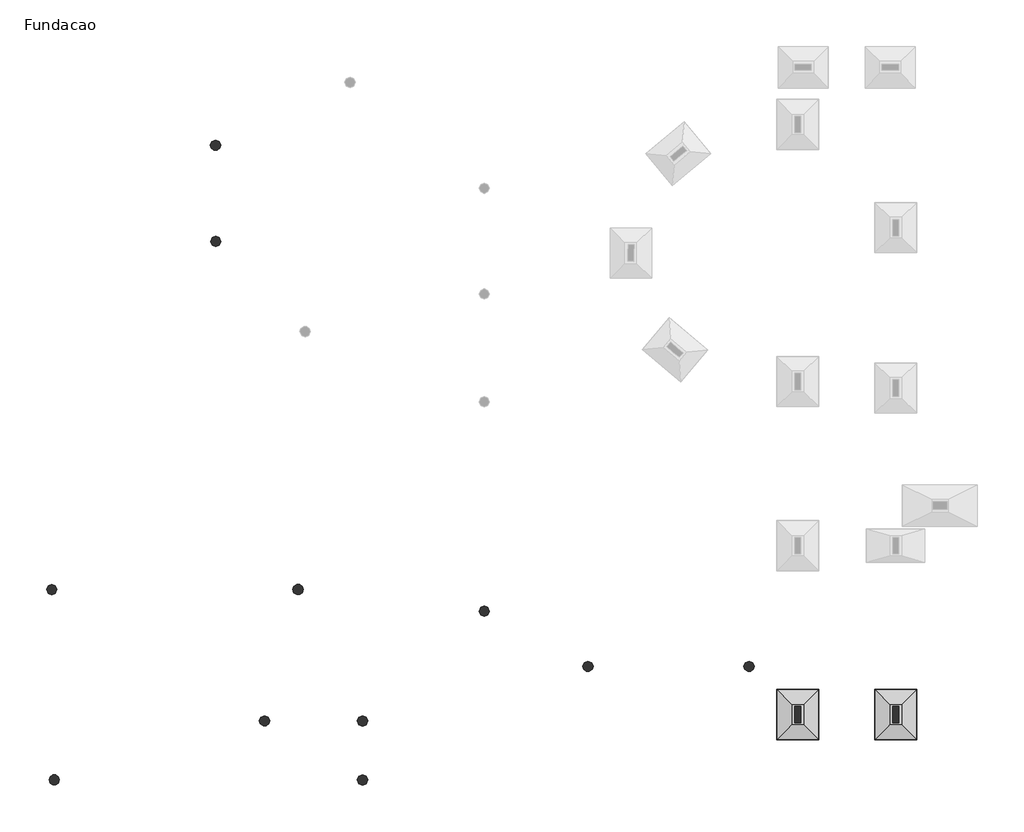
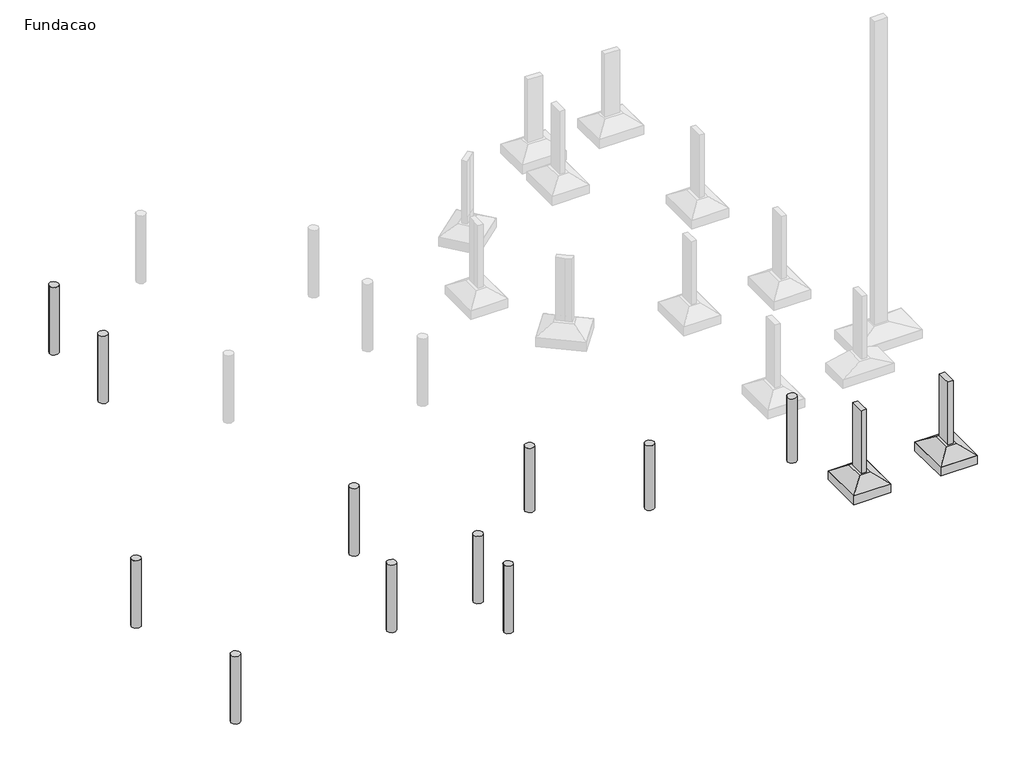
# One storey, part 1 of 2: 13 columns, 2 fasteners.
"""IFC4 building model written with IfcOpenShell, lengths in millimetres."""

import ifcopenshell
import ifcopenshell.guid

model = None  # the IFC model being written
_history = None  # IfcOwnerHistory: only IFC2X3 demands one
_inside = {}  # id of a spatial element -> (the spatial element, [elements in it])
_under = {}  # id of a project, library or spatial element -> (it, [spatial elements below it])
_declared = {}  # id of a project -> (the project, [libraries it declares])
_typed = {}  # id of a type object -> (the type object, [elements of that type])
_made_of = {}  # id of a material, layer set ... -> (it, [elements and type objects made of it])


def new_model(schema):
    """Start an empty IFC model of exactly this schema.

    Asked for "IFC4X3", IfcOpenShell would pick the latest addendum, in which some entities
    have other attributes; the version numbers below select the first issue.
    IFC2X3 requires an IfcOwnerHistory on every rooted entity: one is made here for all.
    """
    global model, _history
    if schema == "IFC4X3":
        model = ifcopenshell.file(schema_version=(4, 3, 0, 0))
    else:
        model = ifcopenshell.file(schema=schema)
    _inside.clear()
    _under.clear()
    _declared.clear()
    _typed.clear()
    _made_of.clear()
    _history = None
    if model.schema == "IFC2X3":
        org = make("IfcOrganization", Name="unknown")
        user = make(
            "IfcPersonAndOrganization",
            ThePerson=make("IfcPerson", FamilyName="unknown"),
            TheOrganization=org,
        )
        app = make(
            "IfcApplication",
            ApplicationDeveloper=org,
            Version="unknown",
            ApplicationFullName="unknown",
            ApplicationIdentifier="unknown",
        )
        _history = make(
            "IfcOwnerHistory",
            OwningUser=user,
            OwningApplication=app,
            ChangeAction="ADDED",
            CreationDate=0,
        )
    return model


def make(cls, **values):
    """One entity of the class cls with the attributes given. An attribute that is None is left unset."""
    return model.create_entity(
        cls, **{name: value for name, value in values.items() if value is not None}
    )


def rooted(cls, **values):
    """An entity with a GlobalId (a new one), such as an element, a storey or a relation."""
    return make(cls, GlobalId=ifcopenshell.guid.new(), OwnerHistory=_history, **values)


def si_unit(unit_type, name, prefix=None):
    """IfcSIUnit, for example si_unit("LENGTHUNIT", "METRE", prefix="MILLI")."""
    return make("IfcSIUnit", UnitType=unit_type, Prefix=prefix, Name=name)


def assignment(units):
    """IfcUnitAssignment: the units of a project."""
    return None if units is None else make("IfcUnitAssignment", Units=units)


def point(xyz):
    """IfcCartesianPoint."""
    return None if xyz is None else make("IfcCartesianPoint", Coordinates=xyz)


def direction(xyz):
    """IfcDirection."""
    return None if xyz is None else make("IfcDirection", DirectionRatios=xyz)


def frame(location, z_axis=None, x_axis=None):
    """IfcAxis2Placement3D, a coordinate frame: its origin and axes. An axis left out is left unset."""
    return make(
        "IfcAxis2Placement3D",
        Location=point(location),
        Axis=direction(z_axis),
        RefDirection=direction(x_axis),
    )


def origin():
    """The frame at (0, 0, 0) with its axes left unset."""
    return frame((0.0, 0.0, 0.0))


def place(relative_to, where):
    """IfcLocalPlacement: puts the frame where relative to a parent placement (None: the world)."""
    return make(
        "IfcLocalPlacement", PlacementRelTo=relative_to, RelativePlacement=where
    )


def context(
    kind, dimensions, precision=None, world=None, true_north=None, identifier=None
):
    """IfcGeometricRepresentationContext, for example the 3D "Model" context."""
    return make(
        "IfcGeometricRepresentationContext",
        ContextIdentifier=identifier,
        ContextType=kind,
        CoordinateSpaceDimension=dimensions,
        Precision=precision,
        WorldCoordinateSystem=world,
        TrueNorth=true_north,
    )


def project(units=None, contexts=None):
    """IfcProject with its units and contexts."""
    return rooted(
        "IfcProject",
        Name="project",
        RepresentationContexts=contexts,
        UnitsInContext=assignment(units),
    )


def spatial(cls, under=None, at=None, **own):
    """A site, building, storey or space (cls), placed at a placement, below another one or the project."""
    s = rooted(cls, ObjectPlacement=at, **own)
    if under is not None:
        _under.setdefault(under.id(), (under, []))[1].append(s)
    return s


def polyline(points):
    """IfcPolyline through the points."""
    return make("IfcPolyline", Points=[point(p) for p in points])


def circle_curve(where, radius):
    """IfcCircle in the frame where."""
    return make("IfcCircle", Position=where, Radius=radius)


def outline(outer, holes=None, kind="AREA"):
    """IfcArbitraryClosedProfileDef: a profile drawn as a closed curve; with holes, ...WithVoids."""
    if holes is None:
        return make("IfcArbitraryClosedProfileDef", ProfileType=kind, OuterCurve=outer)
    return make(
        "IfcArbitraryProfileDefWithVoids",
        ProfileType=kind,
        OuterCurve=outer,
        InnerCurves=holes,
    )


def extrude(swept, where, along, depth):
    """IfcExtrudedAreaSolid: the profile swept, set in the frame where, extruded along a direction by depth."""
    return make(
        "IfcExtrudedAreaSolid",
        SweptArea=swept,
        Position=where,
        ExtrudedDirection=direction(along),
        Depth=depth,
    )


def faces_of(points, faces, orient=None, outer=None):
    """IfcFace entities. A face is a list of loops; a loop is a list of indices into points, from 0.

    orient and outer hold one flag for each loop. By default every Orientation is true, the
    first loop of a face is its IfcFaceOuterBound and the others are IfcFaceBound.
    """
    made = []
    for i, loops in enumerate(faces):
        bounds = []
        for j, loop in enumerate(loops):
            is_outer = j == 0 if outer is None else outer[i][j]
            bounds.append(
                make(
                    "IfcFaceOuterBound" if is_outer else "IfcFaceBound",
                    Bound=make("IfcPolyLoop", Polygon=[points[k] for k in loop]),
                    Orientation=True if orient is None else orient[i][j],
                )
            )
        made.append(make("IfcFace", Bounds=bounds))
    return made


def faceted_brep(points, faces, orient=None, outer=None, voids=None):
    """IfcFacetedBrep: a solid bounded by flat faces; with voids (closed shells), ...WithVoids."""
    shared = [point(p) for p in points]
    hull = make("IfcClosedShell", CfsFaces=faces_of(shared, faces, orient, outer))
    if voids is None:
        return make("IfcFacetedBrep", Outer=hull)
    return make(
        "IfcFacetedBrepWithVoids",
        Outer=hull,
        Voids=[
            make(cls, CfsFaces=faces_of(shared, fs, o, b)) for cls, fs, o, b in voids
        ],
    )


def shape(context_of_items, identifier, shape_type, items):
    """IfcShapeRepresentation: the items that make up one representation, for example the "Body"."""
    return make(
        "IfcShapeRepresentation",
        ContextOfItems=context_of_items,
        RepresentationIdentifier=identifier,
        RepresentationType=shape_type,
        Items=items,
    )


def source(mapping_origin, context_of_items, identifier, shape_type, items):
    """IfcRepresentationMap: a shape defined once, which mapped items show again and again."""
    return make(
        "IfcRepresentationMap",
        MappingOrigin=mapping_origin,
        MappedRepresentation=shape(context_of_items, identifier, shape_type, items),
    )


def transform(
    local_origin,
    x_axis=None,
    y_axis=None,
    z_axis=None,
    scale=None,
    scale2=None,
    scale3=None,
    uniform=True,
):
    """IfcCartesianTransformationOperator3D, or its non-uniform kind. x_axis, y_axis, z_axis: its Axis1, 2, 3."""
    if uniform:
        return make(
            "IfcCartesianTransformationOperator3D",
            Axis1=direction(x_axis),
            Axis2=direction(y_axis),
            LocalOrigin=point(local_origin),
            Scale=scale,
            Axis3=direction(z_axis),
        )
    return make(
        "IfcCartesianTransformationOperator3DnonUniform",
        Axis1=direction(x_axis),
        Axis2=direction(y_axis),
        LocalOrigin=point(local_origin),
        Scale=scale,
        Axis3=direction(z_axis),
        Scale2=scale2,
        Scale3=scale3,
    )


def mapped(mapping_source, mapping_target):
    """IfcMappedItem: shows the shape of a source again, moved by a transform."""
    return make(
        "IfcMappedItem", MappingSource=mapping_source, MappingTarget=mapping_target
    )


def made_of(thing, what):
    """Note that an element or type object is made of a material, layer set ...; save() writes the relation."""
    if what is not None:
        _made_of.setdefault(what.id(), (what, []))[1].append(thing)
    return thing


def element(
    cls,
    number,
    at=None,
    inside=None,
    cuts=None,
    type_object=None,
    material=None,
    context=None,
    identifier="Body",
    shape_type=None,
    held_by="IfcProductDefinitionShape",
    body=None,
    shapes=None,
    **own,
):
    """One element of the class cls, such as IfcWall. Its Tag is "e" and its number.

    at: its placement. inside: the storey or other place that contains it. cuts: it is an
    opening in that element (IfcRelVoidsElement). A single representation is given by context,
    identifier, shape_type and body (its items); several are given by shapes. held_by: the class
    of the entity that holds the representations. save() writes the other relations.
    """
    e = rooted(cls, Tag="e%d" % number, ObjectPlacement=at, **own)
    if body is not None:
        shapes = [shape(context, identifier, shape_type, body)]
    if shapes is not None:
        e.Representation = make(held_by, Representations=shapes)
    if inside is not None:
        _inside.setdefault(inside.id(), (inside, []))[1].append(e)
    if cuts is not None:
        rooted(
            "IfcRelVoidsElement", RelatingBuildingElement=cuts, RelatedOpeningElement=e
        )
    if type_object is not None:
        _typed.setdefault(type_object.id(), (type_object, []))[1].append(e)
    return made_of(e, material)


def aggregate(whole, parts):
    """IfcRelAggregates: a whole, such as a stair, and the parts it consists of."""
    return rooted("IfcRelAggregates", RelatingObject=whole, RelatedObjects=parts)


def save(model, path):
    """Write the relations noted so far, then the file.

    IfcRelAggregates (storeys below a building ...), IfcRelContainedInSpatialStructure (elements
    in a storey), IfcRelDefinesByType, IfcRelAssociatesMaterial and IfcRelDeclares: one each for
    every whole, place, type object, material and project.
    """
    for whole, parts in _under.values():
        aggregate(whole, parts)
    for where, things in _inside.values():
        rooted(
            "IfcRelContainedInSpatialStructure",
            RelatedElements=things,
            RelatingStructure=where,
        )
    for kind, things in _typed.values():
        rooted("IfcRelDefinesByType", RelatedObjects=things, RelatingType=kind)
    for what, things in _made_of.values():
        rooted("IfcRelAssociatesMaterial", RelatedObjects=things, RelatingMaterial=what)
    for by, libraries in _declared.values():
        rooted("IfcRelDeclares", RelatingContext=by, RelatedDefinitions=libraries)
    model.write(path)


def plane_surface(at):
    """IfcPlane: the flat surface through the origin of the frame at, square to its z axis."""
    return make("IfcPlane", Position=at)


def cylinder_surface(at, radius):
    """IfcCylindricalSurface: all points at the distance radius from the z axis of the frame at."""
    return make("IfcCylindricalSurface", Position=at, Radius=radius)


def advanced_brep(points, edges, surfaces, faces):
    """IfcAdvancedBrep: a solid bounded by faces that lie on surfaces and meet in shared edges.

    An edge is (start, end): straight between two places in points (the first is 0);
    or (start, end, curve); or (start, end, curve, False) where it runs against its curve.
    A face is (place in surfaces, loops), or (place, loops, False) where it looks against
    its surface's normal. A loop lists edges by number (the first is 1), with a minus sign
    where the edge is run from its end to its start. The first loop is the outer one.
    """
    corners = [point(p) for p in points]
    vertices = [make("IfcVertexPoint", VertexGeometry=c) for c in corners]
    made = []
    for start, end, *more in edges:
        made.append(
            make(
                "IfcEdgeCurve",
                EdgeStart=vertices[start],
                EdgeEnd=vertices[end],
                EdgeGeometry=more[0] if more else make("IfcPolyline", Points=[corners[start], corners[end]]),
                SameSense=more[1] if len(more) > 1 else True,
            )
        )
    hull = []
    for where, loops, *sense in faces:
        bounds = []
        for j, loop in enumerate(loops):
            ring = [make("IfcOrientedEdge", EdgeElement=made[abs(k) - 1], Orientation=k > 0) for k in loop]
            bounds.append(
                make(
                    "IfcFaceOuterBound" if j == 0 else "IfcFaceBound",
                    Bound=make("IfcEdgeLoop", EdgeList=ring),
                    Orientation=True,
                )
            )
        hull.append(make("IfcAdvancedFace", Bounds=bounds, FaceSurface=surfaces[where], SameSense=sense[0] if sense else True))
    return make("IfcAdvancedBrep", Outer=make("IfcClosedShell", CfsFaces=hull))


def sps1_6b3be553(model_context):
    return source(origin(), model_context, "Body", "SolidModel", [
        faceted_brep([(-55.0, 50.0, 0.0), (-345.0, 50.0, 0.0), (-345.0, -450.0, 0.0), (-55.0, -450.0, 0.0), (300.0, 400.0, -250.0), (300.0, -800.0, -250.0), (-700.0, -800.0, -250.0), (-700.0, 400.0, -250.0)], [[[0, 1, 2, 3]], [[4, 5, 6, 7]], [[4, 7, 1, 0]], [[7, 6, 2, 1]], [[6, 5, 3, 2]], [[5, 4, 0, 3]]]),
        extrude(outline(polyline([(300.0, 400.0), (300.0, -800.0), (-700.0, -800.0), (-700.0, 400.0), (300.0, 400.0)])), frame((0.0, 0.0, -500.0), z_axis=(0.0, 0.0, 1.0), x_axis=(1.0, 0.0, 0.0)), (0.0, 0.0, 1.0), 250.0),
    ])


model = new_model("IFC4")

# Units and contexts
model_context = context("Model", 3, world=origin())
ifc_project = project(units=[si_unit("LENGTHUNIT", "METRE", prefix="MILLI")], contexts=[model_context])

# Site, building, storey
site = spatial("IfcSite", under=ifc_project)
building = spatial("IfcBuilding", under=site)
storey = spatial("IfcBuildingStorey", under=building, Name="Fundacao", Elevation=-1200.0)

# Columns
placement = place(None, origin())
element("IfcColumn", 1, ObjectType="TQS - Pilar circular : TQS - Pilar circular 25.0cm", at=placement, inside=storey, context=model_context, shape_type="AdvancedBrep", body=[
    advanced_brep(
    [(1325.0, -5454.2, -1500.0), (1575.0, -5454.2, -1500.0), (1325.0, -5454.2, 430.0), (1368.7596159, -5359.2, 430.0), (1575.0, -5454.2, 430.0), (1368.759616, -5549.2, 430.0)],
    [
        (0, 1, circle_curve(frame((1450.0, -5454.2, -1500.0), z_axis=(0.0, 0.0, -1.0), x_axis=(1.0, 0.0, 0.0)), 125.0)),
        (1, 0, circle_curve(frame((1450.0, -5454.2, -1500.0), z_axis=(0.0, 0.0, -1.0), x_axis=(1.0, 0.0, 0.0)), 125.0)),
        (2, 3, circle_curve(frame((1450.0, -5454.2, 430.0), z_axis=(0.0, 0.0, -1.0), x_axis=(1.0, 0.0, 0.0)), 125.0)),
        (3, 4, circle_curve(frame((1450.0, -5454.2, 430.0), z_axis=(0.0, 0.0, -1.0), x_axis=(1.0, 0.0, 0.0)), 125.0)),
        (4, 1),
        (0, 2),
        (4, 5, circle_curve(frame((1450.0, -5454.2, 430.0), z_axis=(0.0, 0.0, -1.0), x_axis=(1.0, 0.0, 0.0)), 125.0)),
        (5, 2, circle_curve(frame((1450.0, -5454.2, 430.0), z_axis=(0.0, 0.0, -1.0), x_axis=(1.0, 0.0, 0.0)), 125.0)),
    ],
    [
        plane_surface(frame((1575.0, -5454.2, -1500.0), z_axis=(0.0, 0.0, -1.0), x_axis=(0.0, -1.0, 0.0))),
        cylinder_surface(frame((1450.0, -5454.2, -1500.0), z_axis=(0.0, 0.0, 1.0), x_axis=(1.0, 0.0, 0.0)), 125.0),
        plane_surface(frame((1575.0, -5454.2, 430.0), z_axis=(0.0, 0.0, 1.0), x_axis=(0.0, 1.0, 0.0))),
    ],
    [
        (0, [[1, 2]]),
        (1, [[3, 4, 5, -1, 6]]),
        (1, [[7, 8, -6, -2, -5]]),
        (2, [[-8, -7, -4, -3]]),
    ],
),
])
element("IfcColumn", 2, ObjectType="TQS - Pilar circular : TQS - Pilar circular 25.0cm", at=placement, inside=storey, context=model_context, shape_type="AdvancedBrep", body=[
    advanced_brep(
    [(1325.0, -4039.0, -1500.0), (1575.0, -4039.0, -1500.0), (1325.0, -4039.0, 430.0), (1346.4384241, -3969.0, 430.0), (1575.0, -4039.0, 430.0), (1346.4384241, -4109.0, 430.0)],
    [
        (0, 1, circle_curve(frame((1450.0, -4039.0, -1500.0), z_axis=(0.0, 0.0, -1.0), x_axis=(1.0, 0.0, 0.0)), 125.0)),
        (1, 0, circle_curve(frame((1450.0, -4039.0, -1500.0), z_axis=(0.0, 0.0, -1.0), x_axis=(1.0, 0.0, 0.0)), 125.0)),
        (2, 3, circle_curve(frame((1450.0, -4039.0, 430.0), z_axis=(0.0, 0.0, -1.0), x_axis=(1.0, 0.0, 0.0)), 125.0)),
        (3, 4, circle_curve(frame((1450.0, -4039.0, 430.0), z_axis=(0.0, 0.0, -1.0), x_axis=(1.0, 0.0, 0.0)), 125.0)),
        (4, 1),
        (0, 2),
        (4, 5, circle_curve(frame((1450.0, -4039.0, 430.0), z_axis=(0.0, 0.0, -1.0), x_axis=(1.0, 0.0, 0.0)), 125.0)),
        (5, 2, circle_curve(frame((1450.0, -4039.0, 430.0), z_axis=(0.0, 0.0, -1.0), x_axis=(1.0, 0.0, 0.0)), 125.0)),
    ],
    [
        plane_surface(frame((1575.0, -4039.0, -1500.0), z_axis=(0.0, 0.0, -1.0), x_axis=(0.0, -1.0, 0.0))),
        cylinder_surface(frame((1450.0, -4039.0, -1500.0), z_axis=(0.0, 0.0, 1.0), x_axis=(1.0, 0.0, 0.0)), 125.0),
        plane_surface(frame((1575.0, -4039.0, 430.0), z_axis=(0.0, 0.0, 1.0), x_axis=(0.0, 1.0, 0.0))),
    ],
    [
        (0, [[1, 2]]),
        (1, [[3, 4, 5, -1, 6]]),
        (1, [[7, 8, -6, -2, -5]]),
        (2, [[-8, -7, -4, -3]]),
    ],
),
])
element("IfcColumn", 3, ObjectType="TQS - Pilar circular : TQS - Pilar circular 25.0cm", at=placement, inside=storey, context=model_context, shape_type="AdvancedBrep", body=[
    advanced_brep(
    [(-6065.0, -5454.2, -1500.0), (-5815.0, -5454.2, -1500.0), (-6065.0, -5454.2, 430.0), (-6021.218638, -5359.181408, 430.0), (-5930.0226515, -5329.5988262, 430.0), (-5858.759616, -5359.2, 430.0), (-5815.0, -5454.2, 430.0), (-5858.759616, -5549.2, 430.0), (-6021.218638, -5549.218592, 430.0)],
    [
        (0, 1, circle_curve(frame((-5940.0, -5454.2, -1500.0), z_axis=(0.0, 0.0, -1.0), x_axis=(1.0, 0.0, 0.0)), 125.0)),
        (1, 0, circle_curve(frame((-5940.0, -5454.2, -1500.0), z_axis=(0.0, 0.0, -1.0), x_axis=(1.0, 0.0, 0.0)), 125.0)),
        (2, 3, circle_curve(frame((-5940.0, -5454.2, 430.0), z_axis=(0.0, 0.0, -1.0), x_axis=(1.0, 0.0, 0.0)), 125.0)),
        (3, 4, circle_curve(frame((-5940.0, -5454.2, 430.0), z_axis=(0.0, 0.0, -1.0), x_axis=(1.0, 0.0, 0.0)), 125.0)),
        (4, 5, circle_curve(frame((-5940.0, -5454.2, 430.0), z_axis=(0.0, 0.0, -1.0), x_axis=(1.0, 0.0, 0.0)), 125.0)),
        (5, 6, circle_curve(frame((-5940.0, -5454.2, 430.0), z_axis=(0.0, 0.0, -1.0), x_axis=(1.0, 0.0, 0.0)), 125.0)),
        (6, 1),
        (0, 2),
        (6, 7, circle_curve(frame((-5940.0, -5454.2, 430.0), z_axis=(0.0, 0.0, -1.0), x_axis=(1.0, 0.0, 0.0)), 125.0)),
        (7, 8, circle_curve(frame((-5940.0, -5454.2, 430.0), z_axis=(0.0, 0.0, -1.0), x_axis=(1.0, 0.0, 0.0)), 125.0)),
        (8, 2, circle_curve(frame((-5940.0, -5454.2, 430.0), z_axis=(0.0, 0.0, -1.0), x_axis=(1.0, 0.0, 0.0)), 125.0)),
    ],
    [
        plane_surface(frame((-5815.0, -5454.2, -1500.0), z_axis=(0.0, 0.0, -1.0), x_axis=(0.0, -1.0, 0.0))),
        cylinder_surface(frame((-5940.0, -5454.2, -1500.0), z_axis=(0.0, 0.0, 1.0), x_axis=(1.0, 0.0, 0.0)), 125.0),
        plane_surface(frame((-5815.0, -5454.2, 430.0), z_axis=(0.0, 0.0, 1.0), x_axis=(0.0, 1.0, 0.0))),
    ],
    [
        (0, [[1, 2]]),
        (1, [[3, 4, 5, 6, 7, -1, 8]]),
        (1, [[9, 10, 11, -8, -2, -7]]),
        (2, [[-11, -10, -9, -6, -5, -4, -3]]),
    ],
),
])
element("IfcColumn", 4, ObjectType="TQS - Pilar circular : TQS - Pilar circular 25.0cm", at=placement, inside=storey, context=model_context, shape_type="AdvancedBrep", body=[
    advanced_brep(
    [(4239.0, -1407.1, -1500.0), (4489.0, -1407.1, -1500.0), (4239.0, -1407.1, 340.0), (4269.0, -1325.859616, 340.0), (4459.0, -1325.859616, 340.0), (4489.0, -1407.1, 340.0), (4459.0, -1488.340384, 340.0), (4269.0, -1488.340384, 340.0)],
    [
        (0, 1, circle_curve(frame((4364.0, -1407.1, -1500.0), z_axis=(0.0, 0.0, -1.0), x_axis=(1.0, 0.0, 0.0)), 125.0)),
        (1, 0, circle_curve(frame((4364.0, -1407.1, -1500.0), z_axis=(0.0, 0.0, -1.0), x_axis=(1.0, 0.0, 0.0)), 125.0)),
        (2, 3, circle_curve(frame((4364.0, -1407.1, 340.0), z_axis=(0.0, 0.0, -1.0), x_axis=(1.0, 0.0, 0.0)), 125.0)),
        (3, 4, circle_curve(frame((4364.0, -1407.1, 340.0), z_axis=(0.0, 0.0, -1.0), x_axis=(1.0, 0.0, 0.0)), 125.0)),
        (4, 5, circle_curve(frame((4364.0, -1407.1, 340.0), z_axis=(0.0, 0.0, -1.0), x_axis=(1.0, 0.0, 0.0)), 125.0)),
        (5, 1),
        (0, 2),
        (5, 6, circle_curve(frame((4364.0, -1407.1, 340.0), z_axis=(0.0, 0.0, -1.0), x_axis=(1.0, 0.0, 0.0)), 125.0)),
        (6, 7, circle_curve(frame((4364.0, -1407.1, 340.0), z_axis=(0.0, 0.0, -1.0), x_axis=(1.0, 0.0, 0.0)), 125.0)),
        (7, 2, circle_curve(frame((4364.0, -1407.1, 340.0), z_axis=(0.0, 0.0, -1.0), x_axis=(1.0, 0.0, 0.0)), 125.0)),
    ],
    [
        plane_surface(frame((4489.0, -1407.1, -1500.0), z_axis=(0.0, 0.0, -1.0), x_axis=(0.0, -1.0, 0.0))),
        cylinder_surface(frame((4364.0, -1407.1, -1500.0), z_axis=(0.0, 0.0, 1.0), x_axis=(1.0, 0.0, 0.0)), 125.0),
        plane_surface(frame((4489.0, -1407.1, 340.0), z_axis=(0.0, 0.0, 1.0), x_axis=(0.0, 1.0, 0.0))),
    ],
    [
        (0, [[1, 2]]),
        (1, [[3, 4, 5, 6, -1, 7]]),
        (1, [[8, 9, 10, -7, -2, -6]]),
        (2, [[-10, -9, -8, -5, -4, -3]]),
    ],
),
])
element("IfcColumn", 5, ObjectType="TQS - Pilar circular : TQS - Pilar circular 25.0cm", at=placement, inside=storey, context=model_context, shape_type="AdvancedBrep", body=[
    advanced_brep(
    [(-6125.0, -889.0, -1500.0), (-5875.0, -889.0, -1500.0), (-6125.0, -889.0, 430.0), (-6103.5615759, -819.0, 430.0), (-6069.9643265, -785.4143204, 430.0), (-5929.9854905, -785.448233, 430.0), (-5896.4557386, -818.9743909, 430.0), (-5875.0, -889.0, 430.0), (-5896.4557386, -959.0256091, 430.0), (-5929.9854905, -992.551767, 430.0), (-6069.9643265, -992.5856796, 430.0), (-6103.5615759, -959.0, 430.0)],
    [
        (0, 1, circle_curve(frame((-6000.0, -889.0, -1500.0), z_axis=(0.0, 0.0, -1.0), x_axis=(1.0, 0.0, 0.0)), 125.0)),
        (1, 0, circle_curve(frame((-6000.0, -889.0, -1500.0), z_axis=(0.0, 0.0, -1.0), x_axis=(1.0, 0.0, 0.0)), 125.0)),
        (2, 3, circle_curve(frame((-6000.0, -889.0, 430.0), z_axis=(0.0, 0.0, -1.0), x_axis=(1.0, 0.0, 0.0)), 125.0)),
        (3, 4, circle_curve(frame((-6000.0, -889.0, 430.0), z_axis=(0.0, 0.0, -1.0), x_axis=(1.0, 0.0, 0.0)), 125.0)),
        (4, 5, circle_curve(frame((-6000.0, -889.0, 430.0), z_axis=(0.0, 0.0, -1.0), x_axis=(1.0, 0.0, 0.0)), 125.0)),
        (5, 6, circle_curve(frame((-6000.0, -889.0, 430.0), z_axis=(0.0, 0.0, -1.0), x_axis=(1.0, 0.0, 0.0)), 125.0)),
        (6, 7, circle_curve(frame((-6000.0, -889.0, 430.0), z_axis=(0.0, 0.0, -1.0), x_axis=(1.0, 0.0, 0.0)), 125.0)),
        (7, 1),
        (0, 2),
        (7, 8, circle_curve(frame((-6000.0, -889.0, 430.0), z_axis=(0.0, 0.0, -1.0), x_axis=(1.0, 0.0, 0.0)), 125.0)),
        (8, 9, circle_curve(frame((-6000.0, -889.0, 430.0), z_axis=(0.0, 0.0, -1.0), x_axis=(1.0, 0.0, 0.0)), 125.0)),
        (9, 10, circle_curve(frame((-6000.0, -889.0, 430.0), z_axis=(0.0, 0.0, -1.0), x_axis=(1.0, 0.0, 0.0)), 125.0)),
        (10, 11, circle_curve(frame((-6000.0, -889.0, 430.0), z_axis=(0.0, 0.0, -1.0), x_axis=(1.0, 0.0, 0.0)), 125.0)),
        (11, 2, circle_curve(frame((-6000.0, -889.0, 430.0), z_axis=(0.0, 0.0, -1.0), x_axis=(1.0, 0.0, 0.0)), 125.0)),
    ],
    [
        plane_surface(frame((-5875.0, -889.0, -1500.0), z_axis=(0.0, 0.0, -1.0), x_axis=(0.0, -1.0, 0.0))),
        cylinder_surface(frame((-6000.0, -889.0, -1500.0), z_axis=(0.0, 0.0, 1.0), x_axis=(1.0, 0.0, 0.0)), 125.0),
        plane_surface(frame((-5875.0, -889.0, 430.0), z_axis=(0.0, 0.0, 1.0), x_axis=(0.0, 1.0, 0.0))),
    ],
    [
        (0, [[1, 2]]),
        (1, [[3, 4, 5, 6, 7, 8, -1, 9]]),
        (1, [[10, 11, 12, 13, 14, -9, -2, -8]]),
        (2, [[-14, -13, -12, -11, -10, -7, -6, -5, -4, -3]]),
    ],
),
])
element("IfcColumn", 6, ObjectType="TQS - Pilar circular : TQS - Pilar circular 25.0cm", at=placement, inside=storey, context=model_context, shape_type="AdvancedBrep", body=[
    advanced_brep(
    [(-220.0, -889.0, -1500.0), (30.0, -889.0, -1500.0), (-220.0, -889.0, 430.0), (-198.5615759, -819.0, 430.0), (-139.9762613, -772.3718048, 430.0), (-0.0195064, -807.7368113, 430.0), (30.0, -889.0, 430.0), (-198.5615759, -959.0, 430.0)],
    [
        (0, 1, circle_curve(frame((-95.0, -889.0, -1500.0), z_axis=(0.0, 0.0, -1.0), x_axis=(1.0, 0.0, 0.0)), 125.0)),
        (1, 0, circle_curve(frame((-95.0, -889.0, -1500.0), z_axis=(0.0, 0.0, -1.0), x_axis=(1.0, 0.0, 0.0)), 125.0)),
        (2, 3, circle_curve(frame((-95.0, -889.0, 430.0), z_axis=(0.0, 0.0, -1.0), x_axis=(1.0, 0.0, 0.0)), 125.0)),
        (3, 4, circle_curve(frame((-95.0, -889.0, 430.0), z_axis=(0.0, 0.0, -1.0), x_axis=(1.0, 0.0, 0.0)), 125.0)),
        (4, 5, circle_curve(frame((-95.0, -889.0, 430.0), z_axis=(0.0, 0.0, -1.0), x_axis=(1.0, 0.0, 0.0)), 125.0)),
        (5, 6, circle_curve(frame((-95.0, -889.0, 430.0), z_axis=(0.0, 0.0, -1.0), x_axis=(1.0, 0.0, 0.0)), 125.0)),
        (6, 1),
        (0, 2),
        (6, 7, circle_curve(frame((-95.0, -889.0, 430.0), z_axis=(0.0, 0.0, -1.0), x_axis=(1.0, 0.0, 0.0)), 125.0)),
        (7, 2, circle_curve(frame((-95.0, -889.0, 430.0), z_axis=(0.0, 0.0, -1.0), x_axis=(1.0, 0.0, 0.0)), 125.0)),
    ],
    [
        plane_surface(frame((30.0, -889.0, -1500.0), z_axis=(0.0, 0.0, -1.0), x_axis=(0.0, -1.0, 0.0))),
        cylinder_surface(frame((-95.0, -889.0, -1500.0), z_axis=(0.0, 0.0, 1.0), x_axis=(1.0, 0.0, 0.0)), 125.0),
        plane_surface(frame((30.0, -889.0, 430.0), z_axis=(0.0, 0.0, 1.0), x_axis=(0.0, 1.0, 0.0))),
    ],
    [
        (0, [[1, 2]]),
        (1, [[3, 4, 5, 6, 7, -1, 8]]),
        (1, [[9, 10, -8, -2, -7]]),
        (2, [[-10, -9, -6, -5, -4, -3]]),
    ],
),
])
element("IfcColumn", 7, ObjectType="TQS - Pilar circular : TQS - Pilar circular 25.0cm", at=placement, inside=storey, context=model_context, shape_type="AdvancedBrep", body=[
    advanced_brep(
    [(-2200.0, 9765.575, -1500.0), (-1950.0, 9765.575, -1500.0), (-2200.0, 9765.575, 430.0), (-2159.0, 9858.1438933, 430.0), (-1969.0, 9831.8245283, 430.0), (-1950.0, 9765.575, 430.0), (-1969.0, 9699.3254717, 430.0), (-2159.0, 9673.0061067, 430.0)],
    [
        (0, 1, circle_curve(frame((-2075.0, 9765.575, -1500.0), z_axis=(0.0, 0.0, -1.0), x_axis=(1.0, 0.0, 0.0)), 125.0)),
        (1, 0, circle_curve(frame((-2075.0, 9765.575, -1500.0), z_axis=(0.0, 0.0, -1.0), x_axis=(1.0, 0.0, 0.0)), 125.0)),
        (2, 3, circle_curve(frame((-2075.0, 9765.575, 430.0), z_axis=(0.0, 0.0, -1.0), x_axis=(1.0, 0.0, 0.0)), 125.0)),
        (3, 4, circle_curve(frame((-2075.0, 9765.575, 430.0), z_axis=(0.0, 0.0, -1.0), x_axis=(1.0, 0.0, 0.0)), 125.0)),
        (4, 5, circle_curve(frame((-2075.0, 9765.575, 430.0), z_axis=(0.0, 0.0, -1.0), x_axis=(1.0, 0.0, 0.0)), 125.0)),
        (5, 1),
        (0, 2),
        (5, 6, circle_curve(frame((-2075.0, 9765.575, 430.0), z_axis=(0.0, 0.0, -1.0), x_axis=(1.0, 0.0, 0.0)), 125.0)),
        (6, 7, circle_curve(frame((-2075.0, 9765.575, 430.0), z_axis=(0.0, 0.0, -1.0), x_axis=(1.0, 0.0, 0.0)), 125.0)),
        (7, 2, circle_curve(frame((-2075.0, 9765.575, 430.0), z_axis=(0.0, 0.0, -1.0), x_axis=(1.0, 0.0, 0.0)), 125.0)),
    ],
    [
        plane_surface(frame((-1950.0, 9765.575, -1500.0), z_axis=(0.0, 0.0, -1.0), x_axis=(0.0, -1.0, 0.0))),
        cylinder_surface(frame((-2075.0, 9765.575, -1500.0), z_axis=(0.0, 0.0, 1.0), x_axis=(1.0, 0.0, 0.0)), 125.0),
        plane_surface(frame((-1950.0, 9765.575, 430.0), z_axis=(0.0, 0.0, 1.0), x_axis=(0.0, 1.0, 0.0))),
    ],
    [
        (0, [[1, 2]]),
        (1, [[3, 4, 5, 6, -1, 7]]),
        (1, [[8, 9, 10, -7, -2, -6]]),
        (2, [[-10, -9, -8, -5, -4, -3]]),
    ],
),
])
element("IfcColumn", 8, ObjectType="TQS - Pilar circular : TQS - Pilar circular 25.0cm", at=placement, inside=storey, context=model_context, shape_type="AdvancedBrep", body=[
    advanced_brep(
    [(-2195.0, 7461.075, -1500.0), (-1945.0, 7461.075, -1500.0), (-2195.0, 7461.075, 430.0), (-2159.0, 7548.847433, 430.0), (-1969.0, 7534.7228106, 430.0), (-1945.0, 7461.075, 430.0), (-1969.0, 7387.4271894, 430.0), (-2159.0, 7373.302567, 430.0)],
    [
        (0, 1, circle_curve(frame((-2070.0, 7461.075, -1500.0), z_axis=(0.0, 0.0, -1.0), x_axis=(1.0, 0.0, 0.0)), 125.0)),
        (1, 0, circle_curve(frame((-2070.0, 7461.075, -1500.0), z_axis=(0.0, 0.0, -1.0), x_axis=(1.0, 0.0, 0.0)), 125.0)),
        (2, 3, circle_curve(frame((-2070.0, 7461.075, 430.0), z_axis=(0.0, 0.0, -1.0), x_axis=(1.0, 0.0, 0.0)), 125.0)),
        (3, 4, circle_curve(frame((-2070.0, 7461.075, 430.0), z_axis=(0.0, 0.0, -1.0), x_axis=(1.0, 0.0, 0.0)), 125.0)),
        (4, 5, circle_curve(frame((-2070.0, 7461.075, 430.0), z_axis=(0.0, 0.0, -1.0), x_axis=(1.0, 0.0, 0.0)), 125.0)),
        (5, 1),
        (0, 2),
        (5, 6, circle_curve(frame((-2070.0, 7461.075, 430.0), z_axis=(0.0, 0.0, -1.0), x_axis=(1.0, 0.0, 0.0)), 125.0)),
        (6, 7, circle_curve(frame((-2070.0, 7461.075, 430.0), z_axis=(0.0, 0.0, -1.0), x_axis=(1.0, 0.0, 0.0)), 125.0)),
        (7, 2, circle_curve(frame((-2070.0, 7461.075, 430.0), z_axis=(0.0, 0.0, -1.0), x_axis=(1.0, 0.0, 0.0)), 125.0)),
    ],
    [
        plane_surface(frame((-1945.0, 7461.075, -1500.0), z_axis=(0.0, 0.0, -1.0), x_axis=(0.0, -1.0, 0.0))),
        cylinder_surface(frame((-2070.0, 7461.075, -1500.0), z_axis=(0.0, 0.0, 1.0), x_axis=(1.0, 0.0, 0.0)), 125.0),
        plane_surface(frame((-1945.0, 7461.075, 430.0), z_axis=(0.0, 0.0, 1.0), x_axis=(0.0, 1.0, 0.0))),
    ],
    [
        (0, [[1, 2]]),
        (1, [[3, 4, 5, 6, -1, 7]]),
        (1, [[8, 9, 10, -7, -2, -6]]),
        (2, [[-10, -9, -8, -5, -4, -3]]),
    ],
),
])
element("IfcColumn", 9, ObjectType="TQS - Pilar circular : TQS - Pilar circular 25.0cm", at=placement, inside=storey, context=model_context, shape_type="AdvancedBrep", body=[
    advanced_brep(
    [(6723.0, -2732.3, -1500.0), (6973.0, -2732.3, -1500.0), (6723.0, -2732.3, 340.0), (6951.5615759, -2662.3, 340.0), (6973.0, -2732.3, 340.0), (6951.5615759, -2802.3, 340.0)],
    [
        (0, 1, circle_curve(frame((6848.0, -2732.3, -1500.0), z_axis=(0.0, 0.0, -1.0), x_axis=(1.0, 0.0, 0.0)), 125.0)),
        (1, 0, circle_curve(frame((6848.0, -2732.3, -1500.0), z_axis=(0.0, 0.0, -1.0), x_axis=(1.0, 0.0, 0.0)), 125.0)),
        (2, 3, circle_curve(frame((6848.0, -2732.3, 340.0), z_axis=(0.0, 0.0, -1.0), x_axis=(1.0, 0.0, 0.0)), 125.0)),
        (3, 4, circle_curve(frame((6848.0, -2732.3, 340.0), z_axis=(0.0, 0.0, -1.0), x_axis=(1.0, 0.0, 0.0)), 125.0)),
        (4, 1),
        (0, 2),
        (4, 5, circle_curve(frame((6848.0, -2732.3, 340.0), z_axis=(0.0, 0.0, -1.0), x_axis=(1.0, 0.0, 0.0)), 125.0)),
        (5, 2, circle_curve(frame((6848.0, -2732.3, 340.0), z_axis=(0.0, 0.0, -1.0), x_axis=(1.0, 0.0, 0.0)), 125.0)),
    ],
    [
        plane_surface(frame((6973.0, -2732.3, -1500.0), z_axis=(0.0, 0.0, -1.0), x_axis=(0.0, -1.0, 0.0))),
        cylinder_surface(frame((6848.0, -2732.3, -1500.0), z_axis=(0.0, 0.0, 1.0), x_axis=(1.0, 0.0, 0.0)), 125.0),
        plane_surface(frame((6973.0, -2732.3, 340.0), z_axis=(0.0, 0.0, 1.0), x_axis=(0.0, 1.0, 0.0))),
    ],
    [
        (0, [[1, 2]]),
        (1, [[3, 4, 5, -1, 6]]),
        (1, [[7, 8, -6, -2, -5]]),
        (2, [[-8, -7, -4, -3]]),
    ],
),
])
element("IfcColumn", 10, ObjectType="TQS - Pilar circular : TQS - Pilar circular 25.0cm", at=placement, inside=storey, context=model_context, shape_type="AdvancedBrep", body=[
    advanced_brep(
    [(10587.0, -2732.3, -1500.0), (10837.0, -2732.3, -1500.0), (10587.0, -2732.3, 340.0), (10608.4384241, -2662.3, 340.0), (10837.0, -2732.3, 340.0), (10608.4384241, -2802.3, 340.0)],
    [
        (0, 1, circle_curve(frame((10712.0, -2732.3, -1500.0), z_axis=(0.0, 0.0, -1.0), x_axis=(1.0, 0.0, 0.0)), 125.0)),
        (1, 0, circle_curve(frame((10712.0, -2732.3, -1500.0), z_axis=(0.0, 0.0, -1.0), x_axis=(1.0, 0.0, 0.0)), 125.0)),
        (2, 3, circle_curve(frame((10712.0, -2732.3, 340.0), z_axis=(0.0, 0.0, -1.0), x_axis=(1.0, 0.0, 0.0)), 125.0)),
        (3, 4, circle_curve(frame((10712.0, -2732.3, 340.0), z_axis=(0.0, 0.0, -1.0), x_axis=(1.0, 0.0, 0.0)), 125.0)),
        (4, 1),
        (0, 2),
        (4, 5, circle_curve(frame((10712.0, -2732.3, 340.0), z_axis=(0.0, 0.0, -1.0), x_axis=(1.0, 0.0, 0.0)), 125.0)),
        (5, 2, circle_curve(frame((10712.0, -2732.3, 340.0), z_axis=(0.0, 0.0, -1.0), x_axis=(1.0, 0.0, 0.0)), 125.0)),
    ],
    [
        plane_surface(frame((10837.0, -2732.3, -1500.0), z_axis=(0.0, 0.0, -1.0), x_axis=(0.0, -1.0, 0.0))),
        cylinder_surface(frame((10712.0, -2732.3, -1500.0), z_axis=(0.0, 0.0, 1.0), x_axis=(1.0, 0.0, 0.0)), 125.0),
        plane_surface(frame((10837.0, -2732.3, 340.0), z_axis=(0.0, 0.0, 1.0), x_axis=(0.0, 1.0, 0.0))),
    ],
    [
        (0, [[1, 2]]),
        (1, [[3, 4, 5, -1, 6]]),
        (1, [[7, 8, -6, -2, -5]]),
        (2, [[-8, -7, -4, -3]]),
    ],
),
])
element("IfcColumn", 11, ObjectType="TQS - Pilar circular : TQS - Pilar circular 25.0cm", at=placement, inside=storey, context=model_context, shape_type="AdvancedBrep", body=[
    advanced_brep(
    [(-1023.8, -4039.0, -1500.0), (-773.8, -4039.0, -1500.0), (-1023.8, -4039.0, 430.0), (-968.8, -3935.4384241, 430.0), (-828.8, -3935.4384241, 430.0), (-795.2325043, -3969.0087588, 430.0), (-773.8, -4039.0, 430.0), (-795.2325043, -4108.9912412, 430.0), (-828.8, -4142.5615759, 430.0), (-968.8, -4142.5615759, 430.0)],
    [
        (0, 1, circle_curve(frame((-898.8, -4039.0, -1500.0), z_axis=(0.0, 0.0, -1.0), x_axis=(1.0, 0.0, 0.0)), 125.0)),
        (1, 0, circle_curve(frame((-898.8, -4039.0, -1500.0), z_axis=(0.0, 0.0, -1.0), x_axis=(1.0, 0.0, 0.0)), 125.0)),
        (2, 3, circle_curve(frame((-898.8, -4039.0, 430.0), z_axis=(0.0, 0.0, -1.0), x_axis=(1.0, 0.0, 0.0)), 125.0)),
        (3, 4, circle_curve(frame((-898.8, -4039.0, 430.0), z_axis=(0.0, 0.0, -1.0), x_axis=(1.0, 0.0, 0.0)), 125.0)),
        (4, 5, circle_curve(frame((-898.8, -4039.0, 430.0), z_axis=(0.0, 0.0, -1.0), x_axis=(1.0, 0.0, 0.0)), 125.0)),
        (5, 6, circle_curve(frame((-898.8, -4039.0, 430.0), z_axis=(0.0, 0.0, -1.0), x_axis=(1.0, 0.0, 0.0)), 125.0)),
        (6, 1),
        (0, 2),
        (6, 7, circle_curve(frame((-898.8, -4039.0, 430.0), z_axis=(0.0, 0.0, -1.0), x_axis=(1.0, 0.0, 0.0)), 125.0)),
        (7, 8, circle_curve(frame((-898.8, -4039.0, 430.0), z_axis=(0.0, 0.0, -1.0), x_axis=(1.0, 0.0, 0.0)), 125.0)),
        (8, 9, circle_curve(frame((-898.8, -4039.0, 430.0), z_axis=(0.0, 0.0, -1.0), x_axis=(1.0, 0.0, 0.0)), 125.0)),
        (9, 2, circle_curve(frame((-898.8, -4039.0, 430.0), z_axis=(0.0, 0.0, -1.0), x_axis=(1.0, 0.0, 0.0)), 125.0)),
    ],
    [
        plane_surface(frame((-773.8, -4039.0, -1500.0), z_axis=(0.0, 0.0, -1.0), x_axis=(0.0, -1.0, 0.0))),
        cylinder_surface(frame((-898.8, -4039.0, -1500.0), z_axis=(0.0, 0.0, 1.0), x_axis=(1.0, 0.0, 0.0)), 125.0),
        plane_surface(frame((-773.8, -4039.0, 430.0), z_axis=(0.0, 0.0, 1.0), x_axis=(0.0, 1.0, 0.0))),
    ],
    [
        (0, [[1, 2]]),
        (1, [[3, 4, 5, 6, 7, -1, 8]]),
        (1, [[9, 10, 11, 12, -8, -2, -7]]),
        (2, [[-12, -11, -10, -9, -6, -5, -4, -3]]),
    ],
),
])
element("IfcColumn", 12, ObjectType="TQS - Pilar retangular : 14.0 x 40.0", at=placement, inside=storey, context=model_context, shape_type="Brep", body=[
    faceted_brep([(11806.0, -4085.2, -1450.0), (11806.0, -3685.2, -1450.0), (11946.0, -3685.2, -1450.0), (11946.0, -3945.2, -1450.0), (11946.0, -4085.2, -1450.0), (11806.0, -4085.2, 350.0), (11806.0, -3685.2, 350.0), (11946.0, -3685.2, 350.0), (11946.0, -3685.2, -1250.0), (11946.0, -3945.2, 350.0), (11946.0, -4085.2, 350.0)], [[[0, 1, 2, 3, 4]], [[1, 0, 5, 6]], [[2, 1, 6, 7, 8]], [[7, 9, 10, 4, 3, 2, 8]], [[0, 4, 10, 5]], [[6, 5, 10, 9, 7]]]),
])
element("IfcColumn", 13, ObjectType="TQS - Pilar retangular : 14.0 x 40.0", at=placement, inside=storey, context=model_context, shape_type="Brep", body=[
    faceted_brep([(14154.0, -4085.2, -1450.0), (14154.0, -3945.2, -1450.0), (14154.0, -3685.2, -1450.0), (14294.0, -3685.2, -1450.0), (14294.0, -4085.2, -1450.0), (14154.0, -4085.2, 350.0), (14154.0, -3945.2, 350.0), (14154.0, -3685.2, 350.0), (14294.0, -3685.2, 350.0), (14294.0, -4085.2, 350.0)], [[[0, 1, 2, 3, 4]], [[5, 6, 7, 2, 1, 0]], [[7, 8, 3, 2]], [[8, 9, 4, 3]], [[9, 5, 0, 4]], [[5, 9, 8, 7, 6]]]),
])

# Fasteners
sps1_shape = sps1_6b3be553(model_context)
element("IfcFastener", 14, ObjectType="TQS - Sapata : SPS10", at=placement, inside=storey, context=model_context, shape_type="MappedRepresentation", body=[
    mapped(sps1_shape, transform((14424.0, -3685.2, -1450.0), x_axis=(1.0, 0.0, 0.0), y_axis=(0.0, 1.0, 0.0), z_axis=(0.0, 0.0, 1.0))),
])
element("IfcFastener", 15, ObjectType="TQS - Sapata : SPS9", at=placement, inside=storey, context=model_context, shape_type="MappedRepresentation", body=[
    mapped(sps1_shape, transform((12076.0, -3685.2, -1450.0), x_axis=(1.0, 0.0, 0.0), y_axis=(0.0, 1.0, 0.0), z_axis=(0.0, 0.0, 1.0))),
])

save(model, "model.ifc")

# Revit data of these elements
# Project information
#   Design Option = "Main Model"
#   Project Status = "Status do projeto"
#   Project Address = "RUA SÉRGIO DIAS, LOTE 30, QUADRA G, MONTE MINEIRO/MG"
#   Project Name = "RESIDÊNCIA - ROBERTA VENDRAMINI"
#   Project Number = "034/2017"
#   Zona = "ZER - 01"
#   CA Mín = "0.2"
#   CA Básico = "1"
#   CA Máx = "2"
#   TO Máx = "50"
#   Gabarito Máx = "10"
#   TP Mín = "15"
#   Área Total do Terreno = "620.00 m²"
#   Multifamiliar - Vagas Veículos/Pavto = "0"
#   Multifamiliar - Vagas Bicicletas/Pavto = "0"
#   Multifamiliar - % Vagas PNMR = "0"
#   Multifamiliar - % Vagas Motos = "0"
#   Outros - Área p/ 1 Veículo = "0.00 m²"
#   Outros - Área p/ 1 Bicicleta = "0.00 m²"
#   Outros - Área p/ 1 Utilitário = "0.00 m²"
#   Outros - % Vagas PNMR = "0"
#   Outros - % Vagas Motos = "0"
# Type "TQS - Pilar circular : TQS - Pilar circular 25.0cm"
#   b = 0.25 m
#   Structural Material [instance default] = Concrete - Cast-in-Place Concrete
# Type "TQS - Pilar retangular : 14.0 x 40.0"
#   b = 0.14 m
#   h = 0.40 m
#   Structural Material [instance default] = Concrete - Cast-in-Place Concrete
# Type "TQS - Sapata : SPS10"
#   TY = 0.50 m
#   TX = 0.29 m
#   HS = 0.50 m
#   H0 = 0.25 m
#   EXCYABS = 0.60 m
#   EXCY = 0.00 m
#   EXCXABS = 0.50 m
#   EXCX = 0.00 m
#   DIMY = 1.20 m
#   DIMX = 1.00 m
#   Material estrutural = Concreto - Concreto concretado no local
#   Width = 0
#   Length = 0
# Type "TQS - Sapata : SPS9"
#   TY = 0.50 m
#   TX = 0.29 m
#   HS = 0.50 m
#   H0 = 0.25 m
#   EXCYABS = 0.60 m
#   EXCY = 0.00 m
#   EXCXABS = 0.50 m
#   EXCX = 0.00 m
#   DIMY = 1.20 m
#   DIMX = 1.00 m
#   Material estrutural = Concreto - Concreto concretado no local
#   Width = 0
#   Length = 0
# Element 1 (IfcColumn, "TQS - Pilar circular : TQS - Pilar circular 25.0cm")
#   Uso = "ESTRUTURA"
#   Titulo = "B16"
#   Chave = "B16//0"
#   Tipo Elemento = "Pilar"
#   SHA1 = "82B48CD5E8973EF4D0B8CB7C6B44CDDBAEC6BB1B"
#   Revisão = ""
#   Tipo de carga = ""
#   Divisor de flexao = ""
#   Secao = "C 25"
#   Configuracao = ""
#   Angulo (graus) = ""
#   Detalhamento = ""
#   Casos de vento manual = ""
#   Tipo = ""
#   Alcas = ""
#   Furos = ""
#   Pino = ""
#   Distribuicao = ""
#   Solidarizado = ""
#   Solidarizar na montagem = ""
#   Unir com o próximo = ""
#   Grupo pre moldado = ""
#   Verificado = ""
#   Concreto C = ""
#   Taxa de armadura (kgf/m³) = 0
#   Carga (tf/m²) = 0
#   Carga (tf/m) = 0
#   Carga (tf) = 0
#   Altura = 1.70 m
#   Rebaixo = 0.00 m
#   Altura da fundacao = 0.00 m
#   Largura = 0.00 m
#   Distancia a face = 0.00 m
#   Distancia ao eixo = 0.00 m
#   Resultado de Ensaios fck (MPa) = 0
#   Unique TQS ID = -451
#   Principal = yes
#   Nasce = yes
#   Morre = yes
#   Cabeca de Pilar = no
#   Structural Material = Concrete - Cast-in-Place Concrete
#   Phase Created = CC_AP/ESTR
#   Materials on its faces: "Concrete - Cast-in-Place Concrete"
# Element 2 (IfcColumn, "TQS - Pilar circular : TQS - Pilar circular 25.0cm")
#   Uso = "ESTRUTURA"
#   Titulo = "B14"
#   Chave = "B14//0"
#   Tipo Elemento = "Pilar"
#   SHA1 = "890103B4E596552A9956B4212317A99A4E95CD8C"
#   Revisão = ""
#   Tipo de carga = ""
#   Divisor de flexao = ""
#   Secao = "C 25"
#   Configuracao = ""
#   Angulo (graus) = ""
#   Detalhamento = ""
#   Casos de vento manual = ""
#   Tipo = ""
#   Alcas = ""
#   Furos = ""
#   Pino = ""
#   Distribuicao = ""
#   Solidarizado = ""
#   Solidarizar na montagem = ""
#   Unir com o próximo = ""
#   Grupo pre moldado = ""
#   Verificado = ""
#   Concreto C = ""
#   Taxa de armadura (kgf/m³) = 0
#   Carga (tf/m²) = 0
#   Carga (tf/m) = 0
#   Carga (tf) = 0
#   Altura = 1.70 m
#   Rebaixo = 0.00 m
#   Altura da fundacao = 0.00 m
#   Largura = 0.00 m
#   Distancia a face = 0.00 m
#   Distancia ao eixo = 0.00 m
#   Resultado de Ensaios fck (MPa) = 0
#   Unique TQS ID = -452
#   Principal = yes
#   Nasce = yes
#   Morre = yes
#   Cabeca de Pilar = no
#   Structural Material = Concrete - Cast-in-Place Concrete
#   Phase Created = CC_AP/ESTR
#   Materials on its faces: "Concrete - Cast-in-Place Concrete"
# Element 3 (IfcColumn, "TQS - Pilar circular : TQS - Pilar circular 25.0cm")
#   Uso = "ESTRUTURA"
#   Titulo = "B15"
#   Chave = "B15//0"
#   Tipo Elemento = "Pilar"
#   SHA1 = "ACB1A011FEC3F1C993EA87551150C74DA8F65ED5"
#   Revisão = ""
#   Tipo de carga = ""
#   Divisor de flexao = ""
#   Secao = "C 25"
#   Configuracao = ""
#   Angulo (graus) = ""
#   Detalhamento = ""
#   Casos de vento manual = ""
#   Tipo = ""
#   Alcas = ""
#   Furos = ""
#   Pino = ""
#   Distribuicao = ""
#   Solidarizado = ""
#   Solidarizar na montagem = ""
#   Unir com o próximo = ""
#   Grupo pre moldado = ""
#   Verificado = ""
#   Concreto C = ""
#   Taxa de armadura (kgf/m³) = 0
#   Carga (tf/m²) = 0
#   Carga (tf/m) = 0
#   Carga (tf) = 0
#   Altura = 1.70 m
#   Rebaixo = 0.00 m
#   Altura da fundacao = 0.00 m
#   Largura = 0.00 m
#   Distancia a face = 0.00 m
#   Distancia ao eixo = 0.00 m
#   Resultado de Ensaios fck (MPa) = 0
#   Unique TQS ID = -679
#   Principal = yes
#   Nasce = yes
#   Morre = yes
#   Cabeca de Pilar = no
#   Structural Material = Concrete - Cast-in-Place Concrete
#   Phase Created = CC_AP/ESTR
#   Materials on its faces: "Concrete - Cast-in-Place Concrete"
# Element 4 (IfcColumn, "TQS - Pilar circular : TQS - Pilar circular 25.0cm")
#   Uso = "ESTRUTURA"
#   Titulo = "B10"
#   Chave = "B10//0"
#   Tipo Elemento = "Pilar"
#   SHA1 = "2E6F60FEFD0732D997A2E681D57AE6747D45538C"
#   Revisão = ""
#   Tipo de carga = ""
#   Divisor de flexao = ""
#   Secao = "C 25"
#   Configuracao = ""
#   Angulo (graus) = ""
#   Detalhamento = ""
#   Casos de vento manual = ""
#   Tipo = ""
#   Alcas = ""
#   Furos = ""
#   Pino = ""
#   Distribuicao = ""
#   Solidarizado = ""
#   Solidarizar na montagem = ""
#   Unir com o próximo = ""
#   Grupo pre moldado = ""
#   Verificado = ""
#   Concreto C = ""
#   Taxa de armadura (kgf/m³) = 0
#   Carga (tf/m²) = 0
#   Carga (tf/m) = 0
#   Carga (tf) = 0
#   Altura = 1.70 m
#   Rebaixo = 0.00 m
#   Altura da fundacao = 0.00 m
#   Largura = 0.00 m
#   Distancia a face = 0.00 m
#   Distancia ao eixo = 0.00 m
#   Resultado de Ensaios fck (MPa) = 0
#   Unique TQS ID = -770
#   Principal = yes
#   Nasce = yes
#   Morre = yes
#   Cabeca de Pilar = no
#   Structural Material = Concrete - Cast-in-Place Concrete
#   Phase Created = CC_AP/ESTR
#   Materials on its faces: "Concrete - Cast-in-Place Concrete"
# Element 5 (IfcColumn, "TQS - Pilar circular : TQS - Pilar circular 25.0cm")
#   Uso = "ESTRUTURA"
#   Titulo = "B8"
#   Chave = "B8//0"
#   Tipo Elemento = "Pilar"
#   SHA1 = "E6C3CAD6D8C8E52E07113B10619DE1E217A6EB8C"
#   Revisão = ""
#   Tipo de carga = ""
#   Divisor de flexao = ""
#   Secao = "C 25"
#   Configuracao = ""
#   Angulo (graus) = ""
#   Detalhamento = ""
#   Casos de vento manual = ""
#   Tipo = ""
#   Alcas = ""
#   Furos = ""
#   Pino = ""
#   Distribuicao = ""
#   Solidarizado = ""
#   Solidarizar na montagem = ""
#   Unir com o próximo = ""
#   Grupo pre moldado = ""
#   Verificado = ""
#   Concreto C = ""
#   Taxa de armadura (kgf/m³) = 0
#   Carga (tf/m²) = 0
#   Carga (tf/m) = 0
#   Carga (tf) = 0
#   Altura = 1.70 m
#   Rebaixo = 0.00 m
#   Altura da fundacao = 0.00 m
#   Largura = 0.00 m
#   Distancia a face = 0.00 m
#   Distancia ao eixo = 0.00 m
#   Resultado de Ensaios fck (MPa) = 0
#   Unique TQS ID = -771
#   Principal = yes
#   Nasce = yes
#   Morre = yes
#   Cabeca de Pilar = no
#   Structural Material = Concrete - Cast-in-Place Concrete
#   Phase Created = CC_AP/ESTR
#   Materials on its faces: "Concrete - Cast-in-Place Concrete"
# Element 6 (IfcColumn, "TQS - Pilar circular : TQS - Pilar circular 25.0cm")
#   Uso = "ESTRUTURA"
#   Titulo = "B9"
#   Chave = "B9//0"
#   Tipo Elemento = "Pilar"
#   SHA1 = "9FB2C0593B3F139C3577D329A2270059E79BEF39"
#   Revisão = ""
#   Tipo de carga = ""
#   Divisor de flexao = ""
#   Secao = "C 25"
#   Configuracao = ""
#   Angulo (graus) = ""
#   Detalhamento = ""
#   Casos de vento manual = ""
#   Tipo = ""
#   Alcas = ""
#   Furos = ""
#   Pino = ""
#   Distribuicao = ""
#   Solidarizado = ""
#   Solidarizar na montagem = ""
#   Unir com o próximo = ""
#   Grupo pre moldado = ""
#   Verificado = ""
#   Concreto C = ""
#   Taxa de armadura (kgf/m³) = 0
#   Carga (tf/m²) = 0
#   Carga (tf/m) = 0
#   Carga (tf) = 0
#   Altura = 1.70 m
#   Rebaixo = 0.00 m
#   Altura da fundacao = 0.00 m
#   Largura = 0.00 m
#   Distancia a face = 0.00 m
#   Distancia ao eixo = 0.00 m
#   Resultado de Ensaios fck (MPa) = 0
#   Unique TQS ID = -772
#   Principal = yes
#   Nasce = yes
#   Morre = yes
#   Cabeca de Pilar = no
#   Structural Material = Concrete - Cast-in-Place Concrete
#   Phase Created = CC_AP/ESTR
#   Materials on its faces: "Concrete - Cast-in-Place Concrete"
# Element 7 (IfcColumn, "TQS - Pilar circular : TQS - Pilar circular 25.0cm")
#   Uso = "ESTRUTURA"
#   Titulo = "B2"
#   Chave = "B2//0"
#   Tipo Elemento = "Pilar"
#   SHA1 = "4CE2E912DC9B0318D735B89447CA6954BE93FBBD"
#   Revisão = ""
#   Tipo de carga = ""
#   Divisor de flexao = ""
#   Secao = "C 25"
#   Configuracao = ""
#   Angulo (graus) = ""
#   Detalhamento = ""
#   Casos de vento manual = ""
#   Tipo = ""
#   Alcas = ""
#   Furos = ""
#   Pino = ""
#   Distribuicao = ""
#   Solidarizado = ""
#   Solidarizar na montagem = ""
#   Unir com o próximo = ""
#   Grupo pre moldado = ""
#   Verificado = ""
#   Concreto C = ""
#   Taxa de armadura (kgf/m³) = 0
#   Carga (tf/m²) = 0
#   Carga (tf/m) = 0
#   Carga (tf) = 0
#   Altura = 1.70 m
#   Rebaixo = 0.00 m
#   Altura da fundacao = 0.00 m
#   Largura = 0.00 m
#   Distancia a face = 0.00 m
#   Distancia ao eixo = 0.00 m
#   Resultado de Ensaios fck (MPa) = 0
#   Unique TQS ID = -773
#   Principal = yes
#   Nasce = yes
#   Morre = yes
#   Cabeca de Pilar = no
#   Structural Material = Concrete - Cast-in-Place Concrete
#   Phase Created = CC_AP/ESTR
#   Materials on its faces: "Concrete - Cast-in-Place Concrete"
# Element 8 (IfcColumn, "TQS - Pilar circular : TQS - Pilar circular 25.0cm")
#   Uso = "ESTRUTURA"
#   Titulo = "B4"
#   Chave = "B4//0"
#   Tipo Elemento = "Pilar"
#   SHA1 = "33C063B82A35DA14032FDD3FDBBCC7600ACCE04D"
#   Revisão = ""
#   Tipo de carga = ""
#   Divisor de flexao = ""
#   Secao = "C 25"
#   Configuracao = ""
#   Angulo (graus) = ""
#   Detalhamento = ""
#   Casos de vento manual = ""
#   Tipo = ""
#   Alcas = ""
#   Furos = ""
#   Pino = ""
#   Distribuicao = ""
#   Solidarizado = ""
#   Solidarizar na montagem = ""
#   Unir com o próximo = ""
#   Grupo pre moldado = ""
#   Verificado = ""
#   Concreto C = ""
#   Taxa de armadura (kgf/m³) = 0
#   Carga (tf/m²) = 0
#   Carga (tf/m) = 0
#   Carga (tf) = 0
#   Altura = 1.70 m
#   Rebaixo = 0.00 m
#   Altura da fundacao = 0.00 m
#   Largura = 0.00 m
#   Distancia a face = 0.00 m
#   Distancia ao eixo = 0.00 m
#   Resultado de Ensaios fck (MPa) = 0
#   Unique TQS ID = -774
#   Principal = yes
#   Nasce = yes
#   Morre = yes
#   Cabeca de Pilar = no
#   Structural Material = Concrete - Cast-in-Place Concrete
#   Phase Created = CC_AP/ESTR
#   Materials on its faces: "Concrete - Cast-in-Place Concrete"
# Element 9 (IfcColumn, "TQS - Pilar circular : TQS - Pilar circular 25.0cm")
#   Uso = "ESTRUTURA"
#   Titulo = "B11"
#   Chave = "B11//0"
#   Tipo Elemento = "Pilar"
#   SHA1 = "2558A1ADF8D5268B513975D0933EE7FB03295AA1"
#   Revisão = ""
#   Tipo de carga = ""
#   Divisor de flexao = ""
#   Secao = "C 25"
#   Configuracao = ""
#   Angulo (graus) = ""
#   Detalhamento = ""
#   Casos de vento manual = ""
#   Tipo = ""
#   Alcas = ""
#   Furos = ""
#   Pino = ""
#   Distribuicao = ""
#   Solidarizado = ""
#   Solidarizar na montagem = ""
#   Unir com o próximo = ""
#   Grupo pre moldado = ""
#   Verificado = ""
#   Concreto C = ""
#   Taxa de armadura (kgf/m³) = 0
#   Carga (tf/m²) = 0
#   Carga (tf/m) = 0
#   Carga (tf) = 0
#   Altura = 1.70 m
#   Rebaixo = 0.00 m
#   Altura da fundacao = 0.00 m
#   Largura = 0.00 m
#   Distancia a face = 0.00 m
#   Distancia ao eixo = 0.00 m
#   Resultado de Ensaios fck (MPa) = 0
#   Unique TQS ID = -1336
#   Principal = yes
#   Nasce = yes
#   Morre = yes
#   Cabeca de Pilar = no
#   Structural Material = Concrete - Cast-in-Place Concrete
#   Phase Created = CC_AP/ESTR
#   Materials on its faces: "Concrete - Cast-in-Place Concrete"
# Element 10 (IfcColumn, "TQS - Pilar circular : TQS - Pilar circular 25.0cm")
#   Uso = "ESTRUTURA"
#   Titulo = "B12"
#   Chave = "B12//0"
#   Tipo Elemento = "Pilar"
#   SHA1 = "D0A2F72A927AF64234E8D16B1C0FC8F58D7B701B"
#   Revisão = ""
#   Tipo de carga = ""
#   Divisor de flexao = ""
#   Secao = "C 25"
#   Configuracao = ""
#   Angulo (graus) = ""
#   Detalhamento = ""
#   Casos de vento manual = ""
#   Tipo = ""
#   Alcas = ""
#   Furos = ""
#   Pino = ""
#   Distribuicao = ""
#   Solidarizado = ""
#   Solidarizar na montagem = ""
#   Unir com o próximo = ""
#   Grupo pre moldado = ""
#   Verificado = ""
#   Concreto C = ""
#   Taxa de armadura (kgf/m³) = 0
#   Carga (tf/m²) = 0
#   Carga (tf/m) = 0
#   Carga (tf) = 0
#   Altura = 1.70 m
#   Rebaixo = 0.00 m
#   Altura da fundacao = 0.00 m
#   Largura = 0.00 m
#   Distancia a face = 0.00 m
#   Distancia ao eixo = 0.00 m
#   Resultado de Ensaios fck (MPa) = 0
#   Unique TQS ID = -1337
#   Principal = yes
#   Nasce = yes
#   Morre = yes
#   Cabeca de Pilar = no
#   Structural Material = Concrete - Cast-in-Place Concrete
#   Phase Created = CC_AP/ESTR
#   Materials on its faces: "Concrete - Cast-in-Place Concrete"
# Element 11 (IfcColumn, "TQS - Pilar circular : TQS - Pilar circular 25.0cm")
#   Uso = "ESTRUTURA"
#   Titulo = "B13"
#   Chave = "B13//0"
#   Tipo Elemento = "Pilar"
#   SHA1 = "1494D04942EE98544A552E3EF72B2ED934A4B529"
#   Revisão = ""
#   Tipo de carga = ""
#   Divisor de flexao = ""
#   Secao = "C 25"
#   Configuracao = ""
#   Angulo (graus) = ""
#   Detalhamento = ""
#   Casos de vento manual = ""
#   Tipo = ""
#   Alcas = ""
#   Furos = ""
#   Pino = ""
#   Distribuicao = ""
#   Solidarizado = ""
#   Solidarizar na montagem = ""
#   Unir com o próximo = ""
#   Grupo pre moldado = ""
#   Verificado = ""
#   Concreto C = ""
#   Taxa de armadura (kgf/m³) = 0
#   Carga (tf/m²) = 0
#   Carga (tf/m) = 0
#   Carga (tf) = 0
#   Altura = 1.70 m
#   Rebaixo = 0.00 m
#   Altura da fundacao = 0.00 m
#   Largura = 0.00 m
#   Distancia a face = 0.00 m
#   Distancia ao eixo = 0.00 m
#   Resultado de Ensaios fck (MPa) = 0
#   Unique TQS ID = -450
#   Principal = yes
#   Nasce = yes
#   Morre = yes
#   Cabeca de Pilar = no
#   Structural Material = Concrete - Cast-in-Place Concrete
#   Phase Created = CC_AP/ESTR
#   Materials on its faces: "Concrete - Cast-in-Place Concrete"
# Element 12 (IfcColumn, "TQS - Pilar retangular : 14.0 x 40.0")
